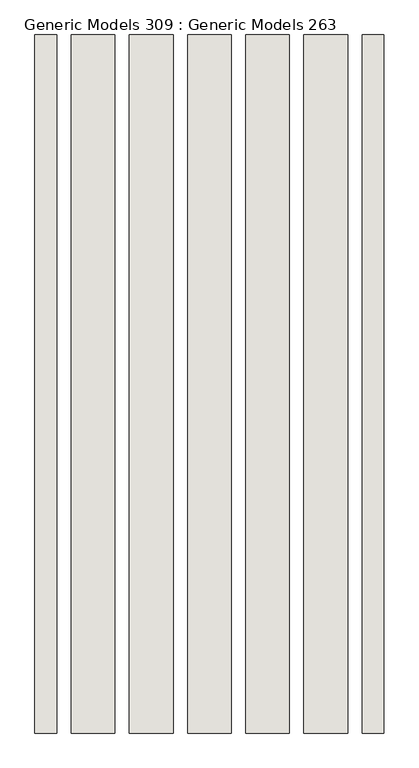
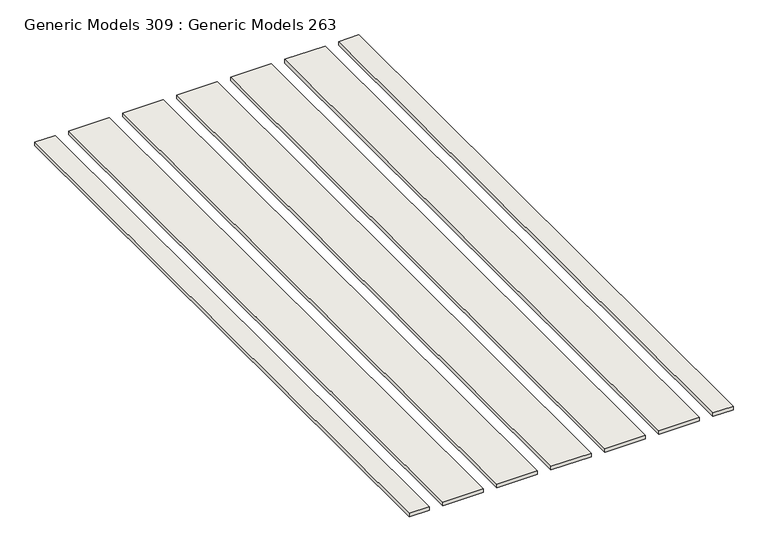
"""IFC4 building model written with IfcOpenShell, lengths in millimetres: wall geometry, Generic Models 309 : Generic Models 263."""

from ifc_helpers import new_model, si_unit, frame, origin, place, context, project, spatial, polyline, outline, extrude, source, transform, mapped, element, save


def generic_models_309_generic_models_263_c606edbc(model_context):
    return source(origin(), model_context, "Body", "SweptSolid", [
        extrude(outline(polyline([(334061.0797726, -94.4486541), (334022.9797726, -94.4486541), (334022.9797726, 1124.7513459), (334061.0797726, 1124.7513459), (334061.0797726, -94.4486541)])), frame((0.0, 0.0, -114.3), z_axis=(0.0, 0.0, 1.0), x_axis=(1.0, 0.0, 0.0)), (0.0, 0.0, 1.0), 7.0017153),
        extrude(outline(polyline([(334632.5797726, -94.4486541), (334594.4797726, -94.4486541), (334594.4797726, 1124.7513459), (334632.5797726, 1124.7513459), (334632.5797726, -94.4486541)])), frame((0.0, 0.0, -114.3), z_axis=(0.0, 0.0, 1.0), x_axis=(1.0, 0.0, 0.0)), (0.0, 0.0, 1.0), 7.0017153),
        extrude(outline(polyline([(334162.6797726, -94.4486541), (334086.4797726, -94.4486541), (334086.4797726, 1124.7513459), (334162.6797726, 1124.7513459), (334162.6797726, -94.4486541)])), frame((0.0, 0.0, -114.3), z_axis=(0.0, 0.0, 1.0), x_axis=(1.0, 0.0, 0.0)), (0.0, 0.0, 1.0), 7.0017153),
        extrude(outline(polyline([(334264.2797726, -94.4486541), (334188.0797726, -94.4486541), (334188.0797726, 1124.7513459), (334264.2797726, 1124.7513459), (334264.2797726, -94.4486541)])), frame((0.0, 0.0, -114.3), z_axis=(0.0, 0.0, 1.0), x_axis=(1.0, 0.0, 0.0)), (0.0, 0.0, 1.0), 7.0017153),
        extrude(outline(polyline([(334365.8797726, -94.4486541), (334289.6797726, -94.4486541), (334289.6797726, 1124.7513459), (334365.8797726, 1124.7513459), (334365.8797726, -94.4486541)])), frame((0.0, 0.0, -114.3), z_axis=(0.0, 0.0, 1.0), x_axis=(1.0, 0.0, 0.0)), (0.0, 0.0, 1.0), 7.0017153),
        extrude(outline(polyline([(334467.4797726, -94.4486541), (334391.2797726, -94.4486541), (334391.2797726, 1124.7513459), (334467.4797726, 1124.7513459), (334467.4797726, -94.4486541)])), frame((0.0, 0.0, -114.3), z_axis=(0.0, 0.0, 1.0), x_axis=(1.0, 0.0, 0.0)), (0.0, 0.0, 1.0), 7.0017153),
        extrude(outline(polyline([(334569.0797726, -94.4486541), (334492.8797726, -94.4486541), (334492.8797726, 1124.7513459), (334569.0797726, 1124.7513459), (334569.0797726, -94.4486541)])), frame((0.0, 0.0, -114.3), z_axis=(0.0, 0.0, 1.0), x_axis=(1.0, 0.0, 0.0)), (0.0, 0.0, 1.0), 7.0017153),
    ])


if __name__ == "__main__":
    model = new_model("IFC4")
    model_context = context("Model", 3, world=origin())
    ifc_project = project(units=[si_unit("LENGTHUNIT", "METRE", prefix="MILLI")], contexts=[model_context])
    site = spatial("IfcSite", under=ifc_project)
    building = spatial("IfcBuilding", under=site)
    placement = place(None, origin())
    generic_models_309_generic_models_263_shape = generic_models_309_generic_models_263_c606edbc(model_context)
    element("IfcWall", 1, ObjectType="Generic Models 309 : Generic Models 263", at=placement, inside=building, context=model_context, shape_type="MappedRepresentation", body=[
        mapped(generic_models_309_generic_models_263_shape, transform((0.0, 0.0, 0.0), x_axis=(1.0, 0.0, 0.0), y_axis=(0.0, 1.0, 0.0), z_axis=(0.0, 0.0, 1.0))),
    ])
    save(model, "model.ifc")

# Revit data of these elements
# Element 1 (IfcWall, "Generic Models 309 : Generic Models 263")
#   Materials on its faces: "EPOXY COATED 6 X 6 X W2.9 X W2.9, PLACED 3\" ABOVE SLAB BASE"
# Materials
#   "EPOXY COATED 6 X 6 X W2.9 X W2.9, PLACED 3\" ABOVE SLAB BASE": class "Miscellaneous", colour RGB 44 44 44, transparency 0, Cost = 0
